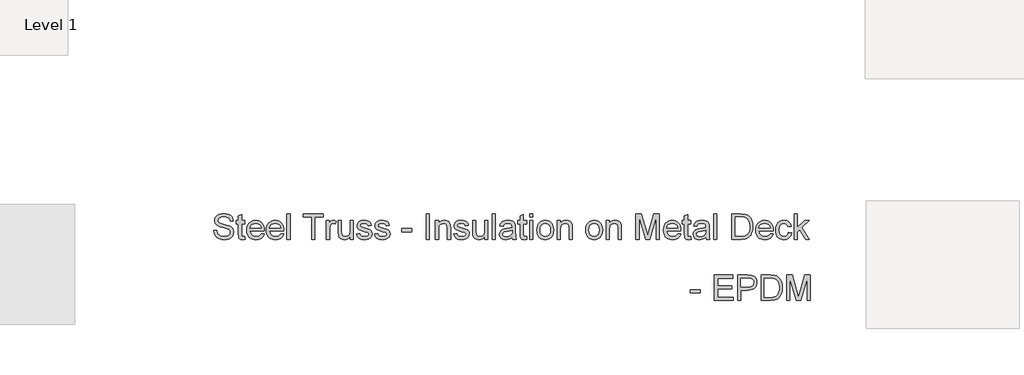
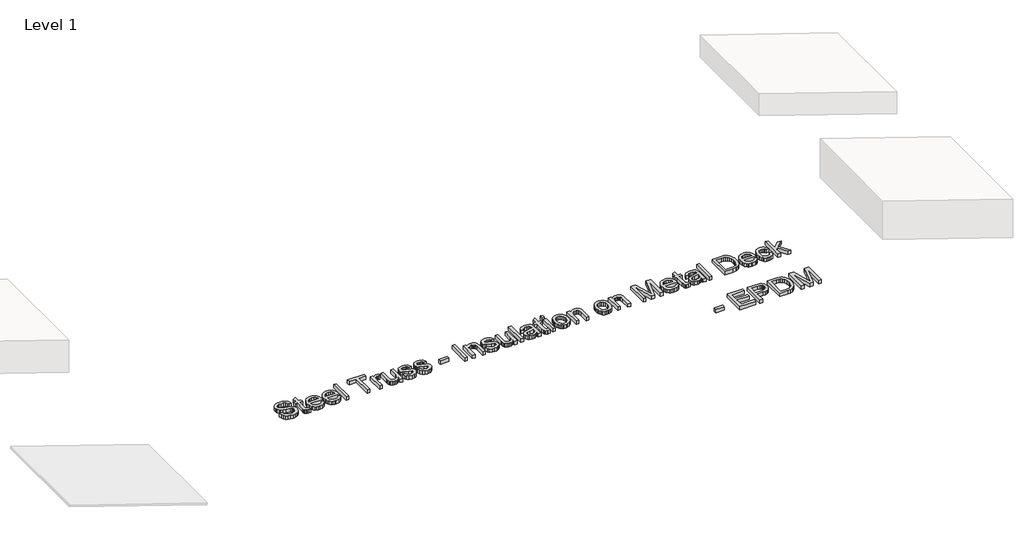
# One storey, part 3 of 42: 1 proxy.
"""IFC4 building model written with IfcOpenShell, lengths in millimetres."""

from ifc_helpers import new_model, si_unit, origin, origin_with_axes, place, context, project, spatial, polyline, outline, extrude, element, save

model = new_model("IFC4")

# Units and contexts
model_context = context("Model", 3, world=origin())
ifc_project = project(units=[si_unit("LENGTHUNIT", "METRE", prefix="MILLI")], contexts=[model_context])

# Site, building, storey
site = spatial("IfcSite", under=ifc_project)
building = spatial("IfcBuilding", under=site)
storey = spatial("IfcBuildingStorey", under=building, Name="Level 1", Elevation=0.0)

# Proxy
placement = place(None, origin())
element("IfcBuildingElementProxy", 1, Name="8\" Arial", ObjectType="8\" Arial", at=placement, inside=storey, context=model_context, shape_type="SweptSolid", body=[
    extrude(outline(polyline([(-9180.0754408, -16969.3529918), (-9142.004554, -16969.3529918), (-9137.6360685, -16990.4797314), (-9129.7356159, -17007.4610572), (-9117.4109099, -17020.9382998), (-9099.769664, -17031.5527902), (-9078.2060758, -17038.4401259), (-9054.1143428, -17040.7359045), (-9032.9039513, -17038.9978049), (-9014.3332404, -17033.7835062), (-8999.2852019, -17025.5298569), (-8988.6428276, -17014.6737056), (-8982.3131708, -17002.2095799), (-8980.2032853, -16989.1320072), (-8981.7833758, -16976.3890419), (-8986.5236473, -16965.3748816), (-8996.1529048, -16955.9779903), (-9012.3999532, -16948.0868324), (-9067.8332463, -16933.5499997), (-9104.2218014, -16923.9300368), (-9127.5048999, -16914.7748065), (-9146.4566914, -16901.9667787), (-9159.8874608, -16886.444713), (-9167.8901545, -16868.5432169), (-9170.5577191, -16848.5968979), (-9167.2581183, -16826.2990323), (-9157.3593159, -16805.5069001), (-9141.1215622, -16787.8842435), (-9118.8051074, -16775.094805), (-9092.0179258, -16767.3151828), (-9062.367992, -16764.7219755), (-9030.2456813, -16767.4360133), (-9002.1386595, -16775.5781268), (-8979.0507487, -16788.9810122), (-8961.9857711, -16807.4773659), (-8951.1853877, -16829.9146512), (-8946.8912594, -16855.1403315), (-8984.9621461, -16855.1403315), (-8991.951723, -16832.4242067), (-9006.5257343, -16816.028444), (-9029.297627, -16806.1017577), (-9060.880848, -16802.7928622), (-9093.207641, -16806.0645791), (-9115.3846761, -16815.8797295), (-9128.2112933, -16830.3236158), (-9132.4868323, -16847.4815398), (-9129.4567764, -16862.1113191), (-9120.3666086, -16873.8783461), (-9098.8773776, -16884.39989), (-9058.2039888, -16895.1445055), (-9016.229349, -16905.3500313), (-8990.836365, -16914.2543061), (-8969.133357, -16928.0661561), (-8953.992372, -16945.1125444), (-8945.0973919, -16965.2075779), (-8942.1323985, -16988.1653636), (-8945.5435351, -17011.634355), (-8955.7769448, -17033.709149), (-8972.4143685, -17052.7074138), (-8995.0375468, -17066.9468177), (-9022.2429876, -17075.8417978), (-9052.6271988, -17078.8067912), (-9089.9266296, -17075.6094316), (-9120.6268588, -17066.0173527), (-9145.0810832, -17049.993376), (-9163.6424994, -17027.5003227), (-9175.5582408, -17000.0996943), (-9180.0754408, -16969.3529918)])), origin_with_axes(), (0.0, 0.0, 1.0), 50.8),
    extrude(outline(polyline([(-8808.8842949, -17042.2974057), (-8804.125434, -17075.1632884), (-8832.6042419, -17078.8067912), (-8850.877524, -17077.2267007), (-8864.503481, -17072.4864292), (-8874.1327385, -17065.1808342), (-8880.4159219, -17055.9047734), (-8883.8735318, -17039.9737432), (-8885.0260684, -17012.7032398), (-8885.0260684, -16888.4523574), (-8913.5792334, -16888.4523574), (-8913.5792334, -16850.3814707), (-8885.0260684, -16850.3814707), (-8885.0260684, -16796.026357), (-8846.9551816, -16773.6448396), (-8846.9551816, -16850.3814707), (-8808.8842949, -16850.3814707), (-8808.8842949, -16888.4523574), (-8846.9551816, -16888.4523574), (-8846.9551816, -17011.5878818), (-8844.9475372, -17031.2181828), (-8838.4412821, -17038.170581), (-8825.4659506, -17040.7359045), (-8808.8842949, -17042.2974057)])), origin_with_axes(), (0.0, 0.0, 1.0), 50.8),
    extrude(outline(polyline([(-8614.2171434, -17007.4238786), (-8576.8898287, -17012.1827394), (-8590.3391874, -17040.3083506), (-8611.8005344, -17061.3328491), (-8640.790548, -17074.4383057), (-8676.8259064, -17078.8067912), (-8700.4482596, -17076.9223009), (-8721.4959947, -17071.26883), (-8739.9691118, -17061.8463785), (-8755.8676108, -17048.6549463), (-8768.652402, -17032.0616723), (-8777.7843957, -17012.433695), (-8783.2635919, -16989.7710144), (-8785.0899906, -16964.0736305), (-8783.2450026, -16937.5048733), (-8777.7100385, -16914.0870024), (-8768.4850983, -16893.8200179), (-8755.570182, -16876.7039197), (-8739.7135089, -16863.1058466), (-8721.6632984, -16853.3929373), (-8701.4195505, -16847.5651917), (-8678.9822652, -16845.6226098), (-8657.267639, -16847.5605444), (-8637.630367, -16853.374348), (-8620.0704493, -16863.0640207), (-8604.5878859, -16876.6295625), (-8591.9494855, -16893.7084821), (-8582.9220566, -16913.938288), (-8577.5055992, -16937.3189803), (-8575.7001135, -16963.8505589), (-8575.9231851, -16974.1118526), (-8747.0191039, -16974.1118526), (-8740.429197, -17002.6092498), (-8725.1209083, -17023.5593911), (-8703.027525, -17036.4417761), (-8676.0823344, -17040.7359045), (-8655.8199972, -17038.7468493), (-8638.7550197, -17032.779684), (-8624.8874017, -17022.4626224), (-8614.2171434, -17007.4238786)]), holes=[polyline([(-8747.0191039, -16936.0409659), (-8613.7710002, -16936.0409659), (-8618.9202364, -16915.9273431), (-8629.0142264, -16901.5392248), (-8651.2098508, -16888.1549286), (-8679.1309796, -16883.6934966), (-8704.7935085, -16887.2533476), (-8726.0131947, -16897.9329005), (-8740.7638044, -16914.5796188), (-8747.0191039, -16936.0409659)])]), origin_with_axes(), (0.0, 0.0, 1.0), 50.8),
    extrude(outline(polyline([(-8381.032962, -17007.4238786), (-8343.7056473, -17012.1827394), (-8357.155006, -17040.3083506), (-8378.616353, -17061.3328491), (-8407.6063666, -17074.4383057), (-8443.641725, -17078.8067912), (-8467.2640782, -17076.9223009), (-8488.3118133, -17071.26883), (-8506.7849304, -17061.8463785), (-8522.6834294, -17048.6549463), (-8535.4682206, -17032.0616723), (-8544.6002143, -17012.433695), (-8550.0794105, -16989.7710144), (-8551.9058092, -16964.0736305), (-8550.0608212, -16937.5048733), (-8544.5258571, -16914.0870024), (-8535.3009169, -16893.8200179), (-8522.3860006, -16876.7039197), (-8506.5293275, -16863.1058466), (-8488.479117, -16853.3929373), (-8468.2353692, -16847.5651917), (-8445.7980838, -16845.6226098), (-8424.0834576, -16847.5605444), (-8404.4461856, -16853.374348), (-8386.8862679, -16863.0640207), (-8371.4037045, -16876.6295625), (-8358.7653041, -16893.7084821), (-8349.7378752, -16913.938288), (-8344.3214178, -16937.3189803), (-8342.5159321, -16963.8505589), (-8342.7390037, -16974.1118526), (-8513.8349225, -16974.1118526), (-8507.2450156, -17002.6092498), (-8491.9367269, -17023.5593911), (-8469.8433436, -17036.4417761), (-8442.898153, -17040.7359045), (-8422.6358158, -17038.7468493), (-8405.5708383, -17032.779684), (-8391.7032203, -17022.4626224), (-8381.032962, -17007.4238786)]), holes=[polyline([(-8513.8349225, -16936.0409659), (-8380.5868188, -16936.0409659), (-8385.736055, -16915.9273431), (-8395.830045, -16901.5392248), (-8418.0256694, -16888.1549286), (-8445.9467982, -16883.6934966), (-8471.6093271, -16887.2533476), (-8492.8290133, -16897.9329005), (-8507.579623, -16914.5796188), (-8513.8349225, -16936.0409659)])]), origin_with_axes(), (0.0, 0.0, 1.0), 50.8),
    extrude(outline(polyline([(-8304.4450453, -17074.0479304), (-8304.4450453, -16769.4808363), (-8266.3741585, -16769.4808363), (-8266.3741585, -17074.0479304), (-8304.4450453, -17074.0479304)])), origin_with_axes(), (0.0, 0.0, 1.0), 50.8),
    extrude(outline(polyline([(-8009.3956729, -17074.0479304), (-8009.3956729, -16807.5517231), (-8109.3317507, -16807.5517231), (-8109.3317507, -16769.4808363), (-7871.3887084, -16769.4808363), (-7871.3887084, -16807.5517231), (-7971.3247862, -16807.5517231), (-7971.3247862, -17074.0479304), (-8009.3956729, -17074.0479304)])), origin_with_axes(), (0.0, 0.0, 1.0), 50.8),
    extrude(outline(polyline([(-7833.3178217, -17074.0479304), (-7833.3178217, -16850.3814707), (-7800.0057958, -16850.3814707), (-7800.0057958, -16883.470425), (-7787.699679, -16864.2862672), (-7776.3602059, -16852.9839727), (-7764.9835542, -16847.4629505), (-7752.5659017, -16845.6226098), (-7733.6048155, -16848.5597193), (-7714.3463006, -16857.3710475), (-7727.0613819, -16891.5010027), (-7740.445678, -16885.6453731), (-7753.8299741, -16883.6934966), (-7765.1973312, -16885.5710159), (-7775.3563837, -16891.2035739), (-7783.5635598, -16900.1636165), (-7789.0752873, -16912.0235901), (-7793.704023, -16933.2897495), (-7795.2469349, -16956.4891961), (-7795.2469349, -17074.0479304), (-7833.3178217, -17074.0479304)])), origin_with_axes(), (0.0, 0.0, 1.0), 50.8),
    extrude(outline(polyline([(-7547.786171, -17074.0479304), (-7547.786171, -17035.6052576), (-7561.5608424, -17054.5059286), (-7577.6034085, -17068.0064078), (-7595.9138691, -17076.1066954), (-7616.4922244, -17078.8067912), (-7635.0350514, -17076.9106826), (-7652.2952166, -17071.2223568), (-7666.7762814, -17062.6712787), (-7676.9818072, -17052.1869134), (-7683.8505536, -17039.4532428), (-7688.3212803, -17024.1542487), (-7690.5519963, -16988.7602212), (-7690.5519963, -16850.3814707), (-7652.4811096, -16850.3814707), (-7652.4811096, -16970.8401358), (-7650.1760363, -17009.6545946), (-7644.6271302, -17022.6020421), (-7635.1187032, -17032.4450766), (-7622.2827914, -17038.6631975), (-7606.7514311, -17040.7359045), (-7590.3277844, -17038.6167242), (-7574.9637278, -17032.2591836), (-7562.2951198, -17022.2488454), (-7553.9578186, -17009.1712728), (-7549.3290829, -16991.2604821), (-7547.786171, -16966.7504898), (-7547.786171, -16850.3814707), (-7509.7152842, -16850.3814707), (-7509.7152842, -17074.0479304), (-7547.786171, -17074.0479304)])), origin_with_axes(), (0.0, 0.0, 1.0), 50.8),
    extrude(outline(polyline([(-7471.6443975, -17007.4238786), (-7433.5735107, -17002.6650177), (-7427.5691668, -17018.9492447), (-7415.9508541, -17030.920754), (-7398.6442157, -17038.2821168), (-7375.5748942, -17040.7359045), (-7352.7844121, -17038.4865991), (-7336.7604354, -17031.7386832), (-7327.2798923, -17021.9607113), (-7324.1197113, -17010.6212382), (-7327.2984816, -17000.9176235), (-7336.8347926, -16993.519082), (-7376.0210374, -16982.6629307), (-7433.3504391, -16964.0364519), (-7447.8593879, -16954.6767393), (-7458.3716371, -16942.2869707), (-7464.7570618, -16927.6571915), (-7466.8855366, -16911.5774469), (-7465.175321, -16896.8268372), (-7460.0446742, -16883.2101748), (-7451.9583286, -16871.2665494), (-7441.3810168, -16861.5350508), (-7417.177748, -16850.2699349), (-7384.423401, -16845.6226098), (-7359.6438639, -16847.4908345), (-7338.098865, -16853.0955085), (-7320.7736372, -16861.8882475), (-7308.6534135, -16873.3206671), (-7300.6228359, -16888.2385805), (-7295.5665462, -16907.4878008), (-7333.637433, -16912.2466617), (-7338.4427671, -16900.2658577), (-7347.9511941, -16891.2407525), (-7362.2556606, -16885.5803106), (-7381.449113, -16883.6934966), (-7403.31013, -16885.4966587), (-7417.8841414, -16890.9061451), (-7426.0820227, -16898.7136511), (-7428.8146499, -16907.7108724), (-7424.2788606, -16918.7900953), (-7410.0766353, -16927.192459), (-7377.2851098, -16935.2973939), (-7321.4056735, -16953.2174792), (-7306.6457691, -16961.7871466), (-7295.4550104, -16973.516995), (-7288.400371, -16988.4442031), (-7286.0488245, -17006.6059493), (-7288.8093356, -17025.3811425), (-7297.0908688, -17043.0409777), (-7310.5774061, -17058.200552), (-7328.9529293, -17069.4749625), (-7351.1485537, -17076.4738341), (-7376.0953946, -17078.8067912), (-7414.4822994, -17074.3081806), (-7442.4963748, -17060.8123487), (-7461.1972108, -17038.4680098), (-7471.6443975, -17007.4238786)])), origin_with_axes(), (0.0, 0.0, 1.0), 50.8),
    extrude(outline(polyline([(-7257.4956594, -17007.4238786), (-7219.4247727, -17002.6650177), (-7213.4204287, -17018.9492447), (-7201.8021161, -17030.920754), (-7184.4954777, -17038.2821168), (-7161.4261561, -17040.7359045), (-7138.6356741, -17038.4865991), (-7122.6116974, -17031.7386832), (-7113.1311543, -17021.9607113), (-7109.9709733, -17010.6212382), (-7113.1497436, -17000.9176235), (-7122.6860546, -16993.519082), (-7161.8722993, -16982.6629307), (-7219.2017011, -16964.0364519), (-7233.7106499, -16954.6767393), (-7244.2228991, -16942.2869707), (-7250.6083237, -16927.6571915), (-7252.7367986, -16911.5774469), (-7251.026583, -16896.8268372), (-7245.8959361, -16883.2101748), (-7237.8095906, -16871.2665494), (-7227.2322788, -16861.5350508), (-7203.0290099, -16850.2699349), (-7170.274663, -16845.6226098), (-7145.4951259, -16847.4908345), (-7123.950127, -16853.0955085), (-7106.6248992, -16861.8882475), (-7094.5046755, -16873.3206671), (-7086.4740978, -16888.2385805), (-7081.4178082, -16907.4878008), (-7119.4886949, -16912.2466617), (-7124.294029, -16900.2658577), (-7133.8024561, -16891.2407525), (-7148.1069226, -16885.5803106), (-7167.300375, -16883.6934966), (-7189.161392, -16885.4966587), (-7203.7354033, -16890.9061451), (-7211.9332847, -16898.7136511), (-7214.6659118, -16907.7108724), (-7210.1301226, -16918.7900953), (-7195.9278973, -16927.192459), (-7163.1363718, -16935.2973939), (-7107.2569354, -16953.2174792), (-7092.4970311, -16961.7871466), (-7081.3062724, -16973.516995), (-7074.251633, -16988.4442031), (-7071.9000865, -17006.6059493), (-7074.6605976, -17025.3811425), (-7082.9421308, -17043.0409777), (-7096.4286681, -17058.200552), (-7114.8041913, -17069.4749625), (-7136.9998157, -17076.4738341), (-7161.9466565, -17078.8067912), (-7200.3335614, -17074.3081806), (-7228.3476368, -17060.8123487), (-7247.0484727, -17038.4680098), (-7257.4956594, -17007.4238786)])), origin_with_axes(), (0.0, 0.0, 1.0), 50.8),
    extrude(outline(polyline([(-6929.1342612, -16983.6295743), (-6929.1342612, -16945.5586876), (-6810.16274, -16945.5586876), (-6810.16274, -16983.6295743), (-6929.1342612, -16983.6295743)])), origin_with_axes(), (0.0, 0.0, 1.0), 50.8),
    extrude(outline(polyline([(-6638.8437496, -17074.0479304), (-6638.8437496, -16769.4808363), (-6600.7728629, -16769.4808363), (-6600.7728629, -17074.0479304), (-6638.8437496, -17074.0479304)])), origin_with_axes(), (0.0, 0.0, 1.0), 50.8),
    extrude(outline(polyline([(-6529.3899502, -17074.0479304), (-6529.3899502, -16850.3814707), (-6491.3190634, -16850.3814707), (-6491.3190634, -16881.611495), (-6478.0927764, -16865.8663577), (-6462.2082194, -16854.6198311), (-6443.6653924, -16847.8719152), (-6422.4642956, -16845.6226098), (-6403.6983971, -16847.4350666), (-6386.512589, -16852.8724369), (-6372.1802386, -16861.2562113), (-6361.9747128, -16871.9078803), (-6350.5608825, -16899.9033663), (-6348.5532381, -16936.7101807), (-6348.5532381, -17074.0479304), (-6386.6241248, -17074.0479304), (-6386.6241248, -16941.8408275), (-6391.0111997, -16908.1570156), (-6397.0806062, -16898.1280882), (-6406.514676, -16890.3484661), (-6418.6070158, -16885.357239), (-6432.6512321, -16883.6934966), (-6454.9490976, -16887.4299459), (-6473.9566571, -16898.6392939), (-6481.5527099, -16907.7898769), (-6486.9784618, -16920.2958286), (-6491.3190634, -16955.3738381), (-6491.3190634, -17074.0479304), (-6529.3899502, -17074.0479304)])), origin_with_axes(), (0.0, 0.0, 1.0), 50.8),
    extrude(outline(polyline([(-6310.4823513, -17007.4238786), (-6272.4114646, -17002.6650177), (-6266.4071206, -17018.9492447), (-6254.788808, -17030.920754), (-6237.4821695, -17038.2821168), (-6214.412848, -17040.7359045), (-6191.622366, -17038.4865991), (-6175.5983893, -17031.7386832), (-6166.1178462, -17021.9607113), (-6162.9576651, -17010.6212382), (-6166.1364355, -17000.9176235), (-6175.6727465, -16993.519082), (-6214.8589912, -16982.6629307), (-6272.188393, -16964.0364519), (-6286.6973418, -16954.6767393), (-6297.209591, -16942.2869707), (-6303.5950156, -16927.6571915), (-6305.7234905, -16911.5774469), (-6304.0132749, -16896.8268372), (-6298.882628, -16883.2101748), (-6290.7962824, -16871.2665494), (-6280.2189706, -16861.5350508), (-6256.0157018, -16850.2699349), (-6223.2613549, -16845.6226098), (-6198.4818178, -16847.4908345), (-6176.9368189, -16853.0955085), (-6159.6115911, -16861.8882475), (-6147.4913674, -16873.3206671), (-6139.4607897, -16888.2385805), (-6134.4045001, -16907.4878008), (-6172.4753868, -16912.2466617), (-6177.2807209, -16900.2658577), (-6186.789148, -16891.2407525), (-6201.0936144, -16885.5803106), (-6220.2870669, -16883.6934966), (-6242.1480839, -16885.4966587), (-6256.7220952, -16890.9061451), (-6264.9199766, -16898.7136511), (-6267.6526037, -16907.7108724), (-6263.1168145, -16918.7900953), (-6248.9145891, -16927.192459), (-6216.1230636, -16935.2973939), (-6160.2436273, -16953.2174792), (-6145.483723, -16961.7871466), (-6134.2929643, -16973.516995), (-6127.2383249, -16988.4442031), (-6124.8867784, -17006.6059493), (-6127.6472895, -17025.3811425), (-6135.9288227, -17043.0409777), (-6149.41536, -17058.200552), (-6167.7908832, -17069.4749625), (-6189.9865076, -17076.4738341), (-6214.9333484, -17078.8067912), (-6253.3202533, -17074.3081806), (-6281.3343287, -17060.8123487), (-6300.0351646, -17038.4680098), (-6310.4823513, -17007.4238786)])), origin_with_axes(), (0.0, 0.0, 1.0), 50.8),
    extrude(outline(polyline([(-5939.2912054, -17074.0479304), (-5939.2912054, -17035.6052576), (-5953.0658769, -17054.5059286), (-5969.1084429, -17068.0064078), (-5987.4189036, -17076.1066954), (-6007.9972589, -17078.8067912), (-6026.5400858, -17076.9106826), (-6043.800251, -17071.2223568), (-6058.2813159, -17062.6712787), (-6068.4868417, -17052.1869134), (-6075.3555881, -17039.4532428), (-6079.8263148, -17024.1542487), (-6082.0570308, -16988.7602212), (-6082.0570308, -16850.3814707), (-6043.986144, -16850.3814707), (-6043.986144, -16970.8401358), (-6041.6810708, -17009.6545946), (-6036.1321647, -17022.6020421), (-6026.6237377, -17032.4450766), (-6013.7878259, -17038.6631975), (-5998.2564656, -17040.7359045), (-5981.8328189, -17038.6167242), (-5966.4687623, -17032.2591836), (-5953.8001542, -17022.2488454), (-5945.4628531, -17009.1712728), (-5940.8341173, -16991.2604821), (-5939.2912054, -16966.7504898), (-5939.2912054, -16850.3814707), (-5901.2203187, -16850.3814707), (-5901.2203187, -17074.0479304), (-5939.2912054, -17074.0479304)])), origin_with_axes(), (0.0, 0.0, 1.0), 50.8),
    extrude(outline(polyline([(-5848.8728494, -17074.0479304), (-5848.8728494, -16769.4808363), (-5810.8019626, -16769.4808363), (-5810.8019626, -17074.0479304), (-5848.8728494, -17074.0479304)])), origin_with_axes(), (0.0, 0.0, 1.0), 50.8),
    extrude(outline(polyline([(-5610.9298071, -17045.4947653), (-5629.1194374, -17061.0911882), (-5647.8481573, -17071.296714), (-5667.5435208, -17076.9292719), (-5688.6330819, -17078.8067912), (-5720.4486691, -17074.2895913), (-5743.9176606, -17060.7379915), (-5758.3894308, -17040.1596362), (-5763.2133542, -17014.5621698), (-5761.3916028, -16998.779854), (-5755.9263485, -16984.4475035), (-5747.4961009, -16972.1785654), (-5736.7793693, -16962.5864865), (-5710.1223129, -16950.0944768), (-5677.182073, -16944.3689724), (-5638.2560784, -16938.3460391), (-5611.1528787, -16931.282105), (-5610.9298071, -16922.8053842), (-5613.5508985, -16905.8147638), (-5621.4141724, -16894.6983623), (-5638.9996504, -16886.444713), (-5663.500348, -16883.6934966), (-5686.1792943, -16885.5245427), (-5702.017378, -16891.0176809), (-5712.8177614, -16901.1767334), (-5720.3836066, -16917.0055225), (-5758.4544933, -16912.2466617), (-5751.8459971, -16891.4266455), (-5741.9843734, -16875.0680613), (-5727.9494517, -16862.5574623), (-5708.8210619, -16853.2814015), (-5685.4264276, -16847.5373077), (-5658.5927728, -16845.6226098), (-5632.8558867, -16847.3142361), (-5612.4541298, -16852.3891151), (-5597.0714839, -16860.0200228), (-5586.3919309, -16869.3797355), (-5579.3094075, -16880.9515748), (-5574.7178504, -16895.2188627), (-5572.8589204, -16928.5308886), (-5572.8589204, -16975.8964255), (-5570.9256332, -17042.0371555), (-5563.3411987, -17074.0479304), (-5601.4120855, -17074.0479304), (-5607.5093759, -17060.8123487), (-5610.9298071, -17045.4947653)]), holes=[polyline([(-5610.9298071, -16969.3529918), (-5672.3488549, -16981.0270723), (-5705.1032018, -16987.19872), (-5719.9374634, -16997.2369421), (-5725.1424674, -17011.8853106), (-5722.3075991, -17023.2061944), (-5713.8029943, -17032.4822552), (-5699.8145459, -17038.6724921), (-5680.528147, -17040.7359045), (-5660.0799168, -17038.4587152), (-5642.011117, -17031.6271474), (-5627.3627485, -17021.5610413), (-5617.175812, -17009.5802374), (-5612.6586121, -16997.2369421), (-5611.1528787, -16980.1347859), (-5610.9298071, -16969.3529918)])]), origin_with_axes(), (0.0, 0.0, 1.0), 50.8),
    extrude(outline(polyline([(-5439.6108167, -17042.2974057), (-5434.8519559, -17075.1632884), (-5463.3307638, -17078.8067912), (-5481.6040458, -17077.2267007), (-5495.2300029, -17072.4864292), (-5504.8592603, -17065.1808342), (-5511.1424438, -17055.9047734), (-5514.6000536, -17039.9737432), (-5515.7525902, -17012.7032398), (-5515.7525902, -16888.4523574), (-5544.3057553, -16888.4523574), (-5544.3057553, -16850.3814707), (-5515.7525902, -16850.3814707), (-5515.7525902, -16796.026357), (-5477.6817035, -16773.6448396), (-5477.6817035, -16850.3814707), (-5439.6108167, -16850.3814707), (-5439.6108167, -16888.4523574), (-5477.6817035, -16888.4523574), (-5477.6817035, -17011.5878818), (-5475.6740591, -17031.2181828), (-5469.167804, -17038.170581), (-5456.1924725, -17040.7359045), (-5439.6108167, -17042.2974057)])), origin_with_axes(), (0.0, 0.0, 1.0), 50.8),
    extrude(outline(polyline([(-5401.53993, -16807.5517231), (-5401.53993, -16769.4808363), (-5363.4690432, -16769.4808363), (-5363.4690432, -16807.5517231), (-5401.53993, -16807.5517231)])), origin_with_axes(), (0.0, 0.0, 1.0), 50.8),
    extrude(outline(polyline([(-5401.53993, -17074.0479304), (-5401.53993, -16850.3814707), (-5363.4690432, -16850.3814707), (-5363.4690432, -17074.0479304), (-5401.53993, -17074.0479304)])), origin_with_axes(), (0.0, 0.0, 1.0), 50.8),
    extrude(outline(polyline([(-5315.8804348, -16962.2147005), (-5313.8216698, -16933.2479235), (-5307.6453748, -16908.2871407), (-5297.3515498, -16887.3323521), (-5282.9401949, -16870.3835577), (-5268.4312461, -16859.550643), (-5252.416564, -16851.8128468), (-5234.8961486, -16847.1701691), (-5215.8699998, -16845.6226098), (-5194.8664143, -16847.5071001), (-5175.8751205, -16853.1605711), (-5158.8961184, -16862.5830226), (-5143.9294081, -16875.7744547), (-5131.7139143, -16892.2887243), (-5122.9885615, -16911.679688), (-5117.7533498, -16933.9473459), (-5116.0082793, -16959.0916981), (-5119.0941031, -16997.5529602), (-5128.3515746, -17026.8311079), (-5143.5111489, -17048.7571875), (-5164.3032811, -17065.1622449), (-5188.9991664, -17075.3956546), (-5215.8699998, -17078.8067912), (-5237.1803088, -17076.9292719), (-5256.348201, -17071.296714), (-5273.3736763, -17061.9091174), (-5288.2567347, -17048.7664821), (-5300.3421035, -17032.0918799), (-5308.9745097, -17012.1083822), (-5314.1539535, -16988.8159891), (-5315.8804348, -16962.2147005)]), holes=[polyline([(-5277.809548, -16962.1403433), (-5273.4038839, -16996.5956112), (-5260.1868914, -17021.1427821), (-5240.2963403, -17035.8376239), (-5215.8699998, -17040.7359045), (-5191.5551952, -17035.8097399), (-5171.7018226, -17021.0312463), (-5158.4848302, -16996.1587626), (-5154.079166, -16960.9506281), (-5158.5127141, -16927.4991825), (-5171.8133584, -16903.286619), (-5191.6946149, -16888.5917772), (-5215.8699998, -16883.6934966), (-5240.2963403, -16888.5731879), (-5260.1868914, -16903.2122618), (-5273.4038839, -16927.7036648), (-5277.809548, -16962.1403433)])]), origin_with_axes(), (0.0, 0.0, 1.0), 50.8),
    extrude(outline(polyline([(-5073.1785317, -17074.0479304), (-5073.1785317, -16850.3814707), (-5035.1076449, -16850.3814707), (-5035.1076449, -16881.611495), (-5021.8813578, -16865.8663577), (-5005.9968008, -16854.6198311), (-4987.4539739, -16847.8719152), (-4966.2528771, -16845.6226098), (-4947.4869785, -16847.4350666), (-4930.3011705, -16852.8724369), (-4915.9688201, -16861.2562113), (-4905.7632943, -16871.9078803), (-4894.349464, -16899.9033663), (-4892.3418196, -16936.7101807), (-4892.3418196, -17074.0479304), (-4930.4127063, -17074.0479304), (-4930.4127063, -16941.8408275), (-4934.7997812, -16908.1570156), (-4940.8691877, -16898.1280882), (-4950.3032575, -16890.3484661), (-4962.3955973, -16885.357239), (-4976.4398136, -16883.6934966), (-4998.7376791, -16887.4299459), (-5017.7452386, -16898.6392939), (-5025.3412913, -16907.7898769), (-5030.7670433, -16920.2958286), (-5035.1076449, -16955.3738381), (-5035.1076449, -17074.0479304), (-5073.1785317, -17074.0479304)])), origin_with_axes(), (0.0, 0.0, 1.0), 50.8),
    extrude(outline(polyline([(-4730.5405509, -16962.2147005), (-4728.4817859, -16933.2479235), (-4722.3054909, -16908.2871407), (-4712.0116659, -16887.3323521), (-4697.6003109, -16870.3835577), (-4683.0913622, -16859.550643), (-4667.0766801, -16851.8128468), (-4649.5562646, -16847.1701691), (-4630.5301159, -16845.6226098), (-4609.5265304, -16847.5071001), (-4590.5352366, -16853.1605711), (-4573.5562345, -16862.5830226), (-4558.5895242, -16875.7744547), (-4546.3740304, -16892.2887243), (-4537.6486776, -16911.679688), (-4532.4134659, -16933.9473459), (-4530.6683954, -16959.0916981), (-4533.7542192, -16997.5529602), (-4543.0116907, -17026.8311079), (-4558.171265, -17048.7571875), (-4578.9633972, -17065.1622449), (-4603.6592825, -17075.3956546), (-4630.5301159, -17078.8067912), (-4651.8404249, -17076.9292719), (-4671.008317, -17071.296714), (-4688.0337923, -17061.9091174), (-4702.9168508, -17048.7664821), (-4715.0022196, -17032.0918799), (-4723.6346258, -17012.1083822), (-4728.8140696, -16988.8159891), (-4730.5405509, -16962.2147005)]), holes=[polyline([(-4692.4696641, -16962.1403433), (-4688.064, -16996.5956112), (-4674.8470075, -17021.1427821), (-4654.9564563, -17035.8376239), (-4630.5301159, -17040.7359045), (-4606.2153113, -17035.8097399), (-4586.3619387, -17021.0312463), (-4573.1449463, -16996.1587626), (-4568.7392821, -16960.9506281), (-4573.1728302, -16927.4991825), (-4586.4734745, -16903.286619), (-4606.354731, -16888.5917772), (-4630.5301159, -16883.6934966), (-4654.9564563, -16888.5731879), (-4674.8470075, -16903.2122618), (-4688.064, -16927.7036648), (-4692.4696641, -16962.1403433)])]), origin_with_axes(), (0.0, 0.0, 1.0), 50.8),
    extrude(outline(polyline([(-4487.8386478, -17074.0479304), (-4487.8386478, -16850.3814707), (-4449.767761, -16850.3814707), (-4449.767761, -16881.611495), (-4436.5414739, -16865.8663577), (-4420.6569169, -16854.6198311), (-4402.11409, -16847.8719152), (-4380.9129932, -16845.6226098), (-4362.1470946, -16847.4350666), (-4344.9612866, -16852.8724369), (-4330.6289362, -16861.2562113), (-4320.4234104, -16871.9078803), (-4309.0095801, -16899.9033663), (-4307.0019357, -16936.7101807), (-4307.0019357, -17074.0479304), (-4345.0728224, -17074.0479304), (-4345.0728224, -16941.8408275), (-4349.4598973, -16908.1570156), (-4355.5293038, -16898.1280882), (-4364.9633736, -16890.3484661), (-4377.0557134, -16885.357239), (-4391.0999297, -16883.6934966), (-4413.3977952, -16887.4299459), (-4432.4053546, -16898.6392939), (-4440.0014074, -16907.7898769), (-4445.4271594, -16920.2958286), (-4449.767761, -16955.3738381), (-4449.767761, -17074.0479304), (-4487.8386478, -17074.0479304)])), origin_with_axes(), (0.0, 0.0, 1.0), 50.8),
    extrude(outline(polyline([(-4130.9240844, -17074.0479304), (-4130.9240844, -16769.4808363), (-4065.4153906, -16769.4808363), (-4003.1040564, -16984.1500747), (-3990.5376895, -17028.9874668), (-3976.9303218, -16980.4322147), (-3915.6599884, -16769.4808363), (-3850.1512946, -16769.4808363), (-3850.1512946, -17074.0479304), (-3888.2221813, -17074.0479304), (-3888.2221813, -16807.5517231), (-3964.7357408, -17074.0479304), (-4016.3396381, -17074.0479304), (-4092.8531976, -16807.5517231), (-4092.8531976, -17074.0479304), (-4130.9240844, -17074.0479304)])), origin_with_axes(), (0.0, 0.0, 1.0), 50.8),
    extrude(outline(polyline([(-3631.6898389, -17007.4238786), (-3594.3625242, -17012.1827394), (-3607.8118828, -17040.3083506), (-3629.2732299, -17061.3328491), (-3658.2632435, -17074.4383057), (-3694.2986019, -17078.8067912), (-3717.9209551, -17076.9223009), (-3738.9686902, -17071.26883), (-3757.4418073, -17061.8463785), (-3773.3403062, -17048.6549463), (-3786.1250974, -17032.0616723), (-3795.2570911, -17012.433695), (-3800.7362874, -16989.7710144), (-3802.5626861, -16964.0736305), (-3800.7176981, -16937.5048733), (-3795.1827339, -16914.0870024), (-3785.9577937, -16893.8200179), (-3773.0428774, -16876.7039197), (-3757.1862044, -16863.1058466), (-3739.1359939, -16853.3929373), (-3718.892246, -16847.5651917), (-3696.4549607, -16845.6226098), (-3674.7403344, -16847.5605444), (-3655.1030625, -16853.374348), (-3637.5431448, -16863.0640207), (-3622.0605814, -16876.6295625), (-3609.422181, -16893.7084821), (-3600.3947521, -16913.938288), (-3594.9782947, -16937.3189803), (-3593.1728089, -16963.8505589), (-3593.3958805, -16974.1118526), (-3764.4917994, -16974.1118526), (-3757.9018924, -17002.6092498), (-3742.5936037, -17023.5593911), (-3720.5002205, -17036.4417761), (-3693.5550299, -17040.7359045), (-3673.2926927, -17038.7468493), (-3656.2277151, -17032.779684), (-3642.3600972, -17022.4626224), (-3631.6898389, -17007.4238786)]), holes=[polyline([(-3764.4917994, -16936.0409659), (-3631.2436957, -16936.0409659), (-3636.3929318, -16915.9273431), (-3646.4869218, -16901.5392248), (-3668.6825463, -16888.1549286), (-3696.6036751, -16883.6934966), (-3722.266204, -16887.2533476), (-3743.4858902, -16897.9329005), (-3758.2364998, -16914.5796188), (-3764.4917994, -16936.0409659)])]), origin_with_axes(), (0.0, 0.0, 1.0), 50.8),
    extrude(outline(polyline([(-3474.2012878, -17042.2974057), (-3469.442427, -17075.1632884), (-3497.9212348, -17078.8067912), (-3516.1945169, -17077.2267007), (-3529.8204739, -17072.4864292), (-3539.4497314, -17065.1808342), (-3545.7329149, -17055.9047734), (-3549.1905247, -17039.9737432), (-3550.3430613, -17012.7032398), (-3550.3430613, -16888.4523574), (-3578.8962264, -16888.4523574), (-3578.8962264, -16850.3814707), (-3550.3430613, -16850.3814707), (-3550.3430613, -16796.026357), (-3512.2721746, -16773.6448396), (-3512.2721746, -16850.3814707), (-3474.2012878, -16850.3814707), (-3474.2012878, -16888.4523574), (-3512.2721746, -16888.4523574), (-3512.2721746, -17011.5878818), (-3510.2645302, -17031.2181828), (-3503.7582751, -17038.170581), (-3490.7829436, -17040.7359045), (-3474.2012878, -17042.2974057)])), origin_with_axes(), (0.0, 0.0, 1.0), 50.8),
    extrude(outline(polyline([(-3293.3645757, -17045.4947653), (-3311.5542059, -17061.0911882), (-3330.2829259, -17071.296714), (-3349.9782894, -17076.9292719), (-3371.0678504, -17078.8067912), (-3402.8834377, -17074.2895913), (-3426.3524292, -17060.7379915), (-3440.8241994, -17040.1596362), (-3445.6481227, -17014.5621698), (-3443.8263713, -16998.779854), (-3438.3611171, -16984.4475035), (-3429.9308695, -16972.1785654), (-3419.2141379, -16962.5864865), (-3392.5570814, -16950.0944768), (-3359.6168415, -16944.3689724), (-3320.690847, -16938.3460391), (-3293.5876473, -16931.282105), (-3293.3645757, -16922.8053842), (-3295.985667, -16905.8147638), (-3303.848941, -16894.6983623), (-3321.434419, -16886.444713), (-3345.9351166, -16883.6934966), (-3368.6140628, -16885.5245427), (-3384.4521466, -16891.0176809), (-3395.25253, -16901.1767334), (-3402.8183751, -16917.0055225), (-3440.8892619, -16912.2466617), (-3434.2807657, -16891.4266455), (-3424.4191419, -16875.0680613), (-3410.3842203, -16862.5574623), (-3391.2558304, -16853.2814015), (-3367.8611962, -16847.5373077), (-3341.0275414, -16845.6226098), (-3315.2906553, -16847.3142361), (-3294.8888983, -16852.3891151), (-3279.5062524, -16860.0200228), (-3268.8266995, -16869.3797355), (-3261.7441761, -16880.9515748), (-3257.152619, -16895.2188627), (-3255.293689, -16928.5308886), (-3255.293689, -16975.8964255), (-3253.3604017, -17042.0371555), (-3245.7759673, -17074.0479304), (-3283.846854, -17074.0479304), (-3289.9441445, -17060.8123487), (-3293.3645757, -17045.4947653)]), holes=[polyline([(-3293.3645757, -16969.3529918), (-3354.7836235, -16981.0270723), (-3387.5379704, -16987.19872), (-3402.3722319, -16997.2369421), (-3407.577236, -17011.8853106), (-3404.7423677, -17023.2061944), (-3396.2377629, -17032.4822552), (-3382.2493145, -17038.6724921), (-3362.9629156, -17040.7359045), (-3342.5146854, -17038.4587152), (-3324.4458856, -17031.6271474), (-3309.7975171, -17021.5610413), (-3299.6105806, -17009.5802374), (-3295.0933806, -16997.2369421), (-3293.5876473, -16980.1347859), (-3293.3645757, -16969.3529918)])]), origin_with_axes(), (0.0, 0.0, 1.0), 50.8),
    extrude(outline(polyline([(-3202.9462197, -17074.0479304), (-3202.9462197, -16769.4808363), (-3164.8753329, -16769.4808363), (-3164.8753329, -17074.0479304), (-3202.9462197, -17074.0479304)])), origin_with_axes(), (0.0, 0.0, 1.0), 50.8),
    extrude(outline(polyline([(-2984.0386208, -17074.0479304), (-2984.0386208, -16769.4808363), (-2878.9718962, -16769.4808363), (-2824.6167825, -16773.8679112), (-2800.3391565, -16782.3260427), (-2779.8537477, -16795.654571), (-2758.7920706, -16818.8540176), (-2743.7905053, -16847.7046114), (-2734.8118734, -16881.6486736), (-2731.818996, -16920.1285249), (-2733.8452297, -16952.8178093), (-2739.9239309, -16981.5847513), (-2749.1814024, -17006.0761543), (-2760.7439471, -17025.9388215), (-2774.053886, -17041.6188962), (-2788.5535402, -17053.5625216), (-2805.2002585, -17062.4203231), (-2824.9513899, -17068.8429263), (-2873.9156066, -17074.0479304), (-2984.0386208, -17074.0479304)]), holes=[polyline([(-2945.967734, -17035.9770436), (-2878.6001102, -17035.9770436), (-2850.7347492, -17034.6014354), (-2829.5987149, -17030.4746108), (-2813.6490954, -17023.8382306), (-2801.3429787, -17014.9339558), (-2788.1166916, -16998.4545412), (-2778.1807107, -16977.1233193), (-2771.9625898, -16950.8473435), (-2769.8898828, -16919.5336673), (-2773.9516449, -16878.0423493), (-2786.1369311, -16847.4071826), (-2804.1406684, -16826.3640948), (-2825.6577833, -16813.6490135), (-2847.5559789, -16809.0760457), (-2879.641111, -16807.5517231), (-2945.967734, -16807.5517231), (-2945.967734, -17035.9770436)])]), origin_with_axes(), (0.0, 0.0, 1.0), 50.8),
    extrude(outline(polyline([(-2527.6341229, -17007.4238786), (-2490.3068082, -17012.1827394), (-2503.7561668, -17040.3083506), (-2525.2175139, -17061.3328491), (-2554.2075275, -17074.4383057), (-2590.2428859, -17078.8067912), (-2613.8652391, -17076.9223009), (-2634.9129742, -17071.26883), (-2653.3860913, -17061.8463785), (-2669.2845902, -17048.6549463), (-2682.0693814, -17032.0616723), (-2691.2013751, -17012.433695), (-2696.6805714, -16989.7710144), (-2698.5069701, -16964.0736305), (-2696.6619821, -16937.5048733), (-2691.1270179, -16914.0870024), (-2681.9020777, -16893.8200179), (-2668.9871614, -16876.7039197), (-2653.1304884, -16863.1058466), (-2635.0802779, -16853.3929373), (-2614.83653, -16847.5651917), (-2592.3992447, -16845.6226098), (-2570.6846184, -16847.5605444), (-2551.0473465, -16853.374348), (-2533.4874288, -16863.0640207), (-2518.0048654, -16876.6295625), (-2505.366465, -16893.7084821), (-2496.3390361, -16913.938288), (-2490.9225787, -16937.3189803), (-2489.1170929, -16963.8505589), (-2489.3401645, -16974.1118526), (-2660.4360834, -16974.1118526), (-2653.8461764, -17002.6092498), (-2638.5378877, -17023.5593911), (-2616.4445045, -17036.4417761), (-2589.4993139, -17040.7359045), (-2569.2369767, -17038.7468493), (-2552.1719991, -17032.779684), (-2538.3043812, -17022.4626224), (-2527.6341229, -17007.4238786)]), holes=[polyline([(-2660.4360834, -16936.0409659), (-2527.1879797, -16936.0409659), (-2532.3372158, -16915.9273431), (-2542.4312058, -16901.5392248), (-2564.6268303, -16888.1549286), (-2592.5479591, -16883.6934966), (-2618.210488, -16887.2533476), (-2639.4301742, -16897.9329005), (-2654.1807838, -16914.5796188), (-2660.4360834, -16936.0409659)])]), origin_with_axes(), (0.0, 0.0, 1.0), 50.8),
    extrude(outline(polyline([(-2308.2803808, -16993.147296), (-2270.2094941, -16997.9061569), (-2280.8239845, -17031.7665671), (-2300.7703036, -17057.3547388), (-2328.170932, -17073.4437781), (-2361.1483505, -17078.8067912), (-2382.5004854, -17076.9362429), (-2401.645141, -17071.3245979), (-2418.5823171, -17061.9718563), (-2433.3120138, -17048.8780179), (-2445.2347262, -17032.2893912), (-2453.7509494, -17012.4522843), (-2458.8606832, -16989.3666971), (-2460.5639279, -16963.0326297), (-2457.6547024, -16929.1536302), (-2448.927026, -16899.7918305), (-2434.2414788, -16876.0811782), (-2413.4586412, -16859.1556204), (-2388.5954522, -16849.0058625), (-2361.6688509, -16845.6226098), (-2329.500067, -16850.2699349), (-2303.7817702, -16864.21191), (-2285.3318898, -16886.7049632), (-2274.9683549, -16917.0055225), (-2313.0392417, -16921.7643833), (-2319.9451667, -16905.1548436), (-2330.6990768, -16893.2483969), (-2344.7061145, -16886.0822217), (-2361.3714221, -16883.6934966), (-2385.9743609, -16888.3965895), (-2405.5024208, -16902.5058684), (-2418.245386, -16926.7834944), (-2422.4930411, -16961.9916289), (-2418.3383325, -16997.6737906), (-2405.8742068, -17022.0350685), (-2386.6993436, -17036.0606955), (-2362.4124229, -17040.7359045), (-2342.6984701, -17037.8173843), (-2326.5350736, -17029.061824), (-2314.7773412, -17014.2461517), (-2308.2803808, -16993.147296)])), origin_with_axes(), (0.0, 0.0, 1.0), 50.8),
    extrude(outline(polyline([(-2236.8974682, -17074.0479304), (-2236.8974682, -16769.4808363), (-2198.8265814, -16769.4808363), (-2198.8265814, -16933.1410351), (-2113.464515, -16850.3814707), (-2060.8196169, -16850.3814707), (-2147.2226841, -16934.1820359), (-2056.0607561, -17074.0479304), (-2100.5263621, -17074.0479304), (-2174.5117768, -16960.6531993), (-2198.8265814, -16984.2244319), (-2198.8265814, -17074.0479304), (-2236.8974682, -17074.0479304)])), origin_with_axes(), (0.0, 0.0, 1.0), 50.8),
    extrude(outline(polyline([(-3478.9601487, -17715.734903), (-3478.9601487, -17677.6640162), (-3359.9886275, -17677.6640162), (-3359.9886275, -17715.734903), (-3478.9601487, -17715.734903)])), origin_with_axes(), (0.0, 0.0, 1.0), 50.8),
    extrude(outline(polyline([(-3193.428498, -17806.1532591), (-3193.428498, -17501.586165), (-2974.5208991, -17501.586165), (-2974.5208991, -17539.6570517), (-3155.3576112, -17539.6570517), (-3155.3576112, -17630.0754078), (-2984.0386208, -17630.0754078), (-2984.0386208, -17668.1462946), (-3155.3576112, -17668.1462946), (-3155.3576112, -17768.0823723), (-2969.7620383, -17768.0823723), (-2969.7620383, -17806.1532591), (-3193.428498, -17806.1532591)])), origin_with_axes(), (0.0, 0.0, 1.0), 50.8),
    extrude(outline(polyline([(-2912.6557081, -17806.1532591), (-2912.6557081, -17501.586165), (-2799.7814775, -17501.586165), (-2754.2748706, -17504.4860958), (-2733.9846495, -17509.9048768), (-2717.2821633, -17518.7254998), (-2703.8328046, -17531.3476346), (-2693.3019661, -17548.1709512), (-2686.4982822, -17568.0150292), (-2684.2303876, -17589.6994478), (-2685.7616812, -17608.3956365), (-2690.355562, -17625.5953865), (-2698.01203, -17641.2986978), (-2708.7310852, -17655.5055704), (-2723.44684, -17667.2818921), (-2743.0934066, -17675.6935504), (-2767.6707851, -17680.7405454), (-2797.1789754, -17682.4228771), (-2874.5848214, -17682.4228771), (-2874.5848214, -17806.1532591), (-2912.6557081, -17806.1532591)]), holes=[polyline([(-2874.5848214, -17644.3519903), (-2794.9482594, -17644.3519903), (-2761.1900903, -17640.8572019), (-2738.8829301, -17630.3728366), (-2726.4466883, -17613.5495199), (-2722.3012743, -17591.0378774), (-2724.7457673, -17573.9357213), (-2732.0792462, -17559.5104243), (-2743.3908354, -17548.654273), (-2757.7696591, -17542.2595538), (-2795.8405458, -17539.6570517), (-2874.5848214, -17539.6570517), (-2874.5848214, -17644.3519903)])]), origin_with_axes(), (0.0, 0.0, 1.0), 50.8),
    extrude(outline(polyline([(-2631.8829183, -17806.1532591), (-2631.8829183, -17501.586165), (-2526.8161937, -17501.586165), (-2472.46108, -17505.9732398), (-2448.183454, -17514.4313714), (-2427.6980452, -17527.7598996), (-2406.6363681, -17550.9593463), (-2391.6348028, -17579.8099401), (-2382.6561708, -17613.7540022), (-2379.6632935, -17652.2338536), (-2381.6895272, -17684.923138), (-2387.7682284, -17713.69008), (-2397.0256999, -17738.181483), (-2408.5882446, -17758.0441502), (-2421.8981835, -17773.7242249), (-2436.3978376, -17785.6678503), (-2453.044556, -17794.5256518), (-2472.7956874, -17800.948255), (-2521.759904, -17806.1532591), (-2631.8829183, -17806.1532591)]), holes=[polyline([(-2593.8120315, -17768.0823723), (-2526.4444077, -17768.0823723), (-2498.5790467, -17766.7067641), (-2477.4430124, -17762.5799394), (-2461.4933929, -17755.9435593), (-2449.1872762, -17747.0392845), (-2435.9609891, -17730.5598699), (-2426.0250081, -17709.2286479), (-2419.8068872, -17682.9526721), (-2417.7341803, -17651.638996), (-2421.7959424, -17610.147678), (-2433.9812286, -17579.5125113), (-2451.9849658, -17558.4694235), (-2473.5020808, -17545.7543422), (-2495.4002764, -17541.1813744), (-2527.4854085, -17539.6570517), (-2593.8120315, -17539.6570517), (-2593.8120315, -17768.0823723)])]), origin_with_axes(), (0.0, 0.0, 1.0), 50.8),
    extrude(outline(polyline([(-2327.3158242, -17806.1532591), (-2327.3158242, -17501.586165), (-2261.8071304, -17501.586165), (-2199.4957962, -17716.2554034), (-2186.9294293, -17761.0927954), (-2173.3220616, -17712.5375434), (-2112.0517282, -17501.586165), (-2046.5430344, -17501.586165), (-2046.5430344, -17806.1532591), (-2084.6139211, -17806.1532591), (-2084.6139211, -17539.6570517), (-2161.1274807, -17806.1532591), (-2212.7313779, -17806.1532591), (-2289.2449375, -17539.6570517), (-2289.2449375, -17806.1532591), (-2327.3158242, -17806.1532591)])), origin_with_axes(), (0.0, 0.0, 1.0), 50.8),
])

save(model, "model.ifc")

# Revit data of these elements
# Element 1 (IfcBuildingElementProxy, "8\" Arial")
#   Phase Created = New Construction
